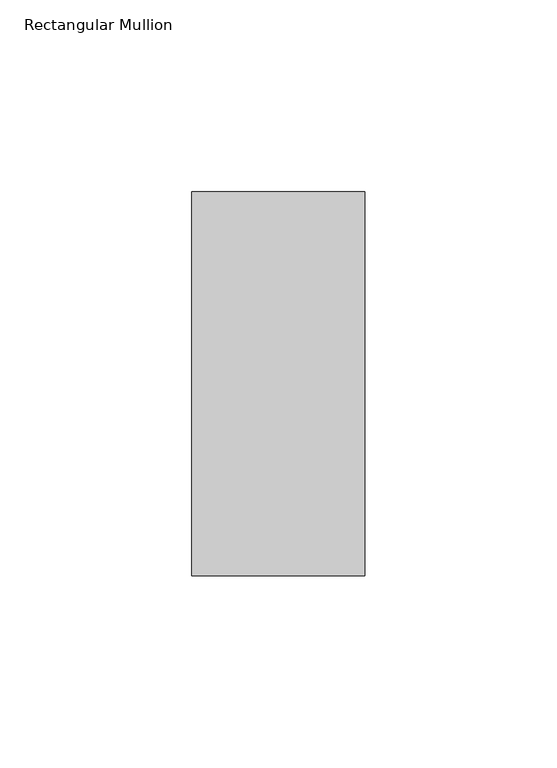
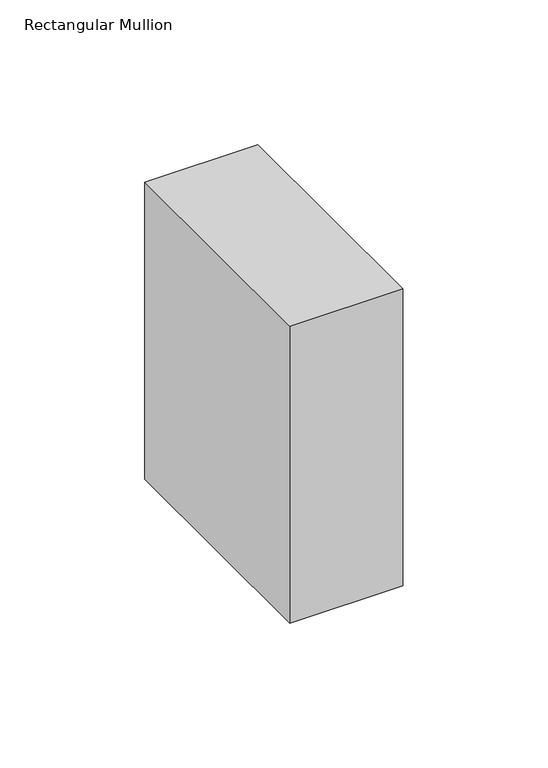
"""IFC4 building model written with IfcOpenShell, lengths in millimetres: member geometry, Rectangular Mullion : 알루미늄_Rectangular Cap_100 x 45."""

from ifc_helpers import new_model, si_unit, frame, origin, place, context, project, spatial, polyline, outline, extrude, source, transform, mapped, element, save


def rectangular_mullion_853566a5(model_context):
    return source(origin(), model_context, "Body", "SweptSolid", [
        extrude(outline(polyline([(0.0, 50.0), (0.0, -50.0), (-45.0, -50.0), (-45.0, 50.0), (0.0, 50.0)])), frame((0.0, 0.0, -125.0), z_axis=(0.0, 0.0, 1.0), x_axis=(1.0, 0.0, 0.0)), (0.0, 0.0, 1.0), 125.0),
    ])


if __name__ == "__main__":
    model = new_model("IFC4")
    model_context = context("Model", 3, world=origin())
    ifc_project = project(units=[si_unit("LENGTHUNIT", "METRE", prefix="MILLI")], contexts=[model_context])
    site = spatial("IfcSite", under=ifc_project)
    building = spatial("IfcBuilding", under=site)
    placement = place(None, origin())
    rectangular_mullion_shape = rectangular_mullion_853566a5(model_context)
    element("IfcMember", 1, ObjectType="Rectangular Mullion : 알루미늄_Rectangular Cap_100 x 45", at=placement, inside=building, context=model_context, shape_type="MappedRepresentation", body=[
        mapped(rectangular_mullion_shape, transform((0.0, 0.0, 0.0), x_axis=(1.0, 0.0, 0.0), y_axis=(0.0, 1.0, 0.0), z_axis=(0.0, 0.0, 1.0))),
    ])
    save(model, "model.ifc")

# Revit data of these elements
# Type "Rectangular Mullion : 알루미늄_Rectangular Cap_100 x 45"
#   built-in parameter 1007304 = 0.328084 (stored number, unit not read)
#   built-in parameter 1007301 = 0.0738189 (stored number, unit not read)
#   built-in parameter 1007300 = 0.0738189 (stored number, unit not read)
# Element 1 (IfcMember, "Rectangular Mullion : 알루미늄_Rectangular Cap_100 x 45")
#   Materials on its faces: "00_Metal_Stainless Steel"
# Materials
#   "00_Metal_Stainless Steel": class "Metal", colour RGB 148 148 148, transparency 0, Description = "Steel", Cost = 0
